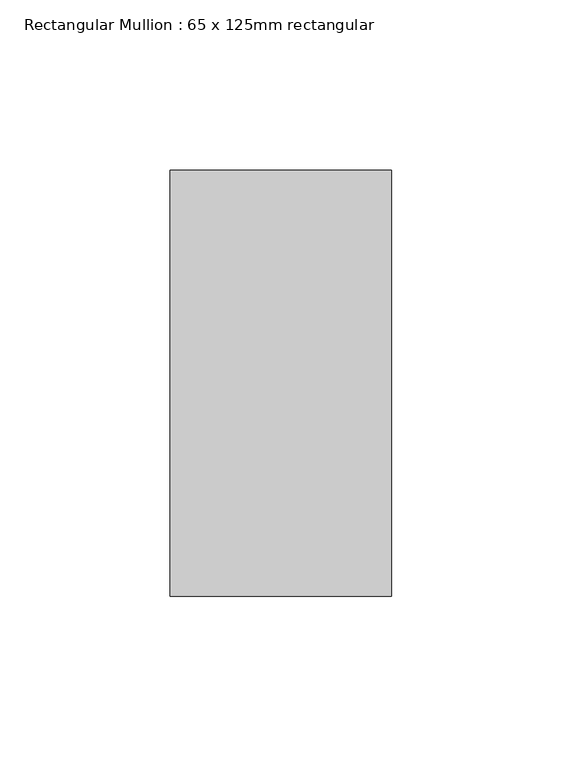
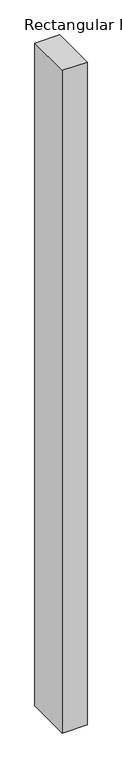
"""IFC4 building model written with IfcOpenShell, lengths in millimetres: member geometry, Rectangular Mullion : 65 x 125mm rectangular."""

from ifc_helpers import new_model, si_unit, frame, origin, place, context, project, spatial, polyline, outline, extrude, source, transform, mapped, element, save


def rectangular_mullion_65_x_125mm_rectangular_abf36099(model_context):
    return source(origin(), model_context, "Body", "SweptSolid", [
        extrude(outline(polyline([(0.0, 62.5), (0.0, -62.5), (-65.0, -62.5), (-65.0, 62.5), (0.0, 62.5)])), frame((0.0, 0.0, -1844.3827623), z_axis=(0.0, 0.0, 1.0), x_axis=(1.0, 0.0, 0.0)), (0.0, 0.0, 1.0), 1844.3827623),
    ])


if __name__ == "__main__":
    model = new_model("IFC4")
    model_context = context("Model", 3, world=origin())
    ifc_project = project(units=[si_unit("LENGTHUNIT", "METRE", prefix="MILLI")], contexts=[model_context])
    site = spatial("IfcSite", under=ifc_project)
    building = spatial("IfcBuilding", under=site)
    placement = place(None, origin())
    rectangular_mullion_65_x_125mm_rectangular_shape = rectangular_mullion_65_x_125mm_rectangular_abf36099(model_context)
    element("IfcMember", 1, ObjectType="Rectangular Mullion : 65 x 125mm rectangular", at=placement, inside=building, context=model_context, shape_type="MappedRepresentation", body=[
        mapped(rectangular_mullion_65_x_125mm_rectangular_shape, transform((0.0, 0.0, 0.0), x_axis=(1.0, 0.0, 0.0), y_axis=(0.0, 1.0, 0.0), z_axis=(0.0, 0.0, 1.0))),
    ])
    save(model, "model.ifc")

# Revit data of these elements
# Type "Rectangular Mullion : 65 x 125mm rectangular"
#   built-in parameter 1007304 = 0.410105 (stored number, unit not read)
#   built-in parameter 1007301 = 0.106627 (stored number, unit not read)
#   built-in parameter 1007300 = 0.106627 (stored number, unit not read)
# Element 1 (IfcMember, "Rectangular Mullion : 65 x 125mm rectangular")
#   Materials on its faces: "Aluminum"
# Materials
#   "Aluminum": class "Metal", colour RGB 244 245 246, transparency 0, Description = "Aluminum 6061", Cost = 0
